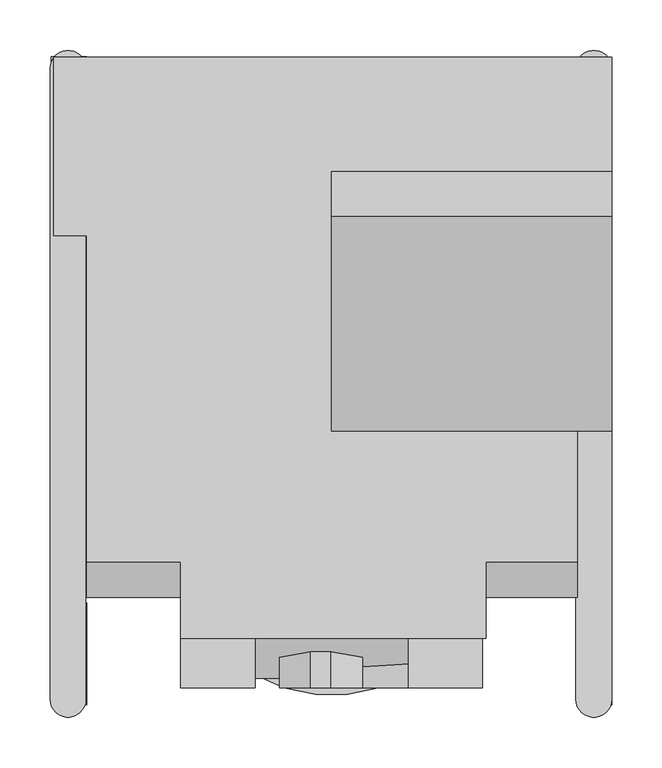
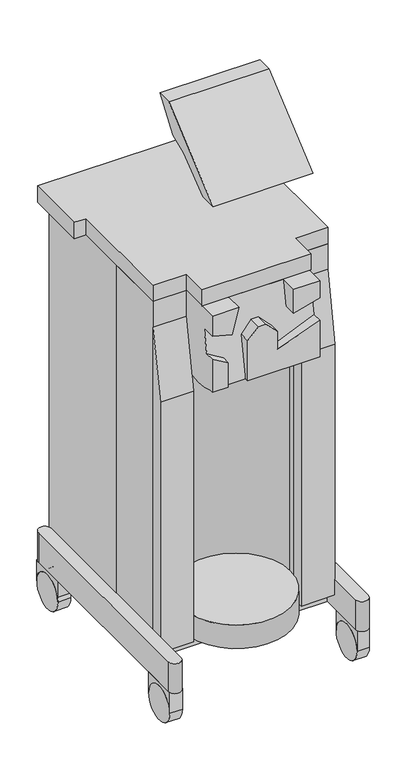
"""IFC4 building model written with IfcOpenShell, lengths in millimetres: proxy geometry, TB010 - CUSA : TB010 - CUSA."""

from ifc_helpers import new_model, si_unit, point, frame, frame_2d, origin, place, context, project, spatial, polyline, circle_curve, trimmed, segment, composite_curve, outline, extrude, faceted_brep, source, transform, mapped, element, save
from ifc_brep_helpers import plane_surface, cylinder_surface, revolved_surface, advanced_brep


def specialty_equipment_cd9e3837(model_context):
    return source(origin(), model_context, "Body", "SolidModel", [
        advanced_brep(
        [(31.190048, -304.8, 1006.9380598), (31.190048, -304.8, 1060.4753847), (-0.5345673, -304.8, 1092.2), (-21.0690363, -304.8, 1092.2), (-51.8302413, -304.8, 1061.4387949), (-51.8302413, -304.8, 943.2729477), (150.5310109, -304.8, 943.2729477), (150.5310109, -304.8, 1050.374618), (31.190048, -283.9074285, 1006.9380598), (31.190048, -274.4673537, 1060.4753847), (-0.5345673, -268.873448, 1092.2), (-21.0690363, -268.873448, 1092.2), (-51.8302413, -274.2974784, 1061.4387949), (-51.8302413, -295.1333055, 943.2729477), (150.5310109, -295.1333055, 943.2729477), (150.5310109, -179.2373321, 943.2729477), (150.5310109, -179.2373321, 1168.4), (150.5310109, -304.8, 1168.4), (150.5310109, -304.8, 1117.6), (150.5310109, -264.3947427, 1117.6), (150.5310109, -276.2483913, 1050.374618), (-150.5310109, -179.2373321, 1168.4), (-150.5310109, -179.2373321, 943.2729477), (-150.5310109, -295.1333055, 943.2729477), (-150.5310109, -304.8, 943.2729477), (-150.5310109, -304.8, 1041.4), (-150.5310109, -277.8308586, 1041.4), (-150.5310109, -265.83553, 1109.4288894), (-150.5310109, -304.8, 1109.4288894), (-150.5310109, -304.8, 1168.4), (76.9274629, -267.8722654, 1097.8779888), (76.9274629, -255.4373321, 1168.4), (-76.2, -255.4373321, 1168.4), (-95.9220112, -268.4156235, 1094.796452), (-106.5369204, -282.309564, 1016.0), (-106.5369204, -295.1333055, 943.2729477), (-76.2, -304.8, 1168.4), (76.9274629, -304.8, 1168.4), (76.9274629, -304.8, 1097.8779888), (-95.9220112, -304.8, 1094.796452), (-106.5369204, -304.8, 1016.0), (-106.5369204, -304.8, 943.2729477)],
        [
            (0, 1),
            (1, 2),
            (2, 3),
            (3, 4),
            (4, 5),
            (5, 6),
            (6, 7),
            (7, 0),
            (0, 8),
            (8, 9),
            (9, 1),
            (9, 10),
            (10, 2),
            (10, 11),
            (11, 3),
            (11, 12),
            (12, 4),
            (12, 13),
            (13, 5),
            (13, 14),
            (14, 6),
            (14, 15, circle_curve(frame((150.5310109, -237.1853188, 1091.5120177), z_axis=(1.0, 0.0, 0.0), x_axis=(0.0, 1.0, 0.0)), 159.1627816)),
            (15, 16),
            (16, 17),
            (17, 18),
            (18, 19),
            (19, 20),
            (20, 7),
            (20, 8),
            (21, 22),
            (22, 23, circle_curve(frame((-150.5310109, -237.1853188, 1091.5120177), z_axis=(-1.0, 0.0, 0.0), x_axis=(0.0, 1.0, 0.0)), 159.1627816)),
            (23, 24),
            (24, 25),
            (25, 26),
            (26, 27),
            (27, 28),
            (28, 29),
            (29, 21),
            (19, 30),
            (30, 31),
            (31, 32),
            (32, 33),
            (33, 27),
            (26, 34),
            (34, 35),
            (35, 13),
            (35, 23),
            (22, 15),
            (21, 16),
            (29, 36),
            (36, 32),
            (31, 37),
            (37, 17),
            (38, 18),
            (37, 38),
            (38, 30),
            (39, 36),
            (28, 39),
            (39, 33),
            (40, 25),
            (24, 41),
            (41, 40),
            (40, 34),
            (35, 41),
        ],
        [
            plane_surface(frame((31.190048, -304.8, 1006.9380598), z_axis=(0.0, -1.0, 0.0), x_axis=(0.0, 0.0, 1.0))),
            plane_surface(frame((31.190048, -304.8, 1006.9380598), z_axis=(1.0, 0.0, 0.0), x_axis=(0.0, 1.0, 0.0))),
            plane_surface(frame((31.190048, -304.8, 1060.4753847), z_axis=(0.7071067811865496, 0.0, 0.7071067811865456), x_axis=(0.0, 1.0, 0.0))),
            plane_surface(frame((-0.5345673, -304.8, 1092.2), z_axis=(0.0, 0.0, 1.0), x_axis=(0.0, 1.0, 0.0))),
            plane_surface(frame((-21.0690363, -304.8, 1092.2), z_axis=(-0.707106781186545, 0.0, 0.7071067811865501), x_axis=(0.0, 1.0, 0.0))),
            plane_surface(frame((-51.8302413, -304.8, 1061.4387949), z_axis=(-1.0, 0.0, 0.0), x_axis=(0.0, 1.0, 0.0))),
            plane_surface(frame((-51.8302413, -304.8, 943.2729477), z_axis=(0.0, 0.0, -1.0), x_axis=(0.0, 1.0, 0.0))),
            plane_surface(frame((150.5310109, -304.8, 943.2729477), z_axis=(1.0, 0.0, 0.0), x_axis=(0.0, 1.0, 0.0))),
            plane_surface(frame((150.5310109, -304.8, 1050.374618), z_axis=(-0.3420201433256685, 0.0, 0.9396926207859085), x_axis=(0.0, 1.0, 0.0))),
            plane_surface(frame((-150.5310109, -255.4373321, 1168.4), z_axis=(-1.0, 0.0, 0.0), x_axis=(0.0, 0.17364817766693152, 0.9848077530122079))),
            plane_surface(frame((150.5310109, -255.4373321, 1168.4), z_axis=(0.0, -0.9848077530122079, 0.17364817766693152), x_axis=(-1.0, 0.0, 0.0))),
            cylinder_surface(frame((-150.5310109, -237.1853188, 1091.5120177), z_axis=(1.0, 0.0, 0.0), x_axis=(0.0, 1.0, 0.0)), 159.1627816),
            plane_surface(frame((150.5310109, -179.2373321, 943.2729477), z_axis=(0.0, 1.0, 0.0), x_axis=(-1.0, 0.0, 0.0))),
            plane_surface(frame((150.5310109, -179.2373321, 1168.4), z_axis=(0.0, 0.0, 1.0), x_axis=(-1.0, 0.0, 0.0))),
            plane_surface(frame((150.5310109, -304.8, 1117.6), z_axis=(0.0, -1.0000000000000002, 0.0), x_axis=(0.9659258262890681, 0.0, 0.2588190451025219))),
            plane_surface(frame((76.9274629, -304.8, 1097.8779888), z_axis=(0.2588190451025219, 0.0, -0.9659258262890681), x_axis=(0.0, 1.0, 0.0))),
            plane_surface(frame((76.9274629, -304.8, 1168.4), z_axis=(-1.0, 0.0, 0.0), x_axis=(0.0, 1.0, 0.0))),
            plane_surface(frame((-76.2, -304.8, 1168.4), z_axis=(0.0, -1.0000000000000002, 0.0), x_axis=(0.2588190451025218, 0.0, 0.9659258262890681))),
            plane_surface(frame((-95.9220112, -304.8, 1094.796452), z_axis=(0.9659258262890681, 0.0, -0.2588190451025218), x_axis=(0.0, 1.0, 0.0))),
            plane_surface(frame((-150.5310109, -304.8, 1109.4288894), z_axis=(-0.25881904510252624, 0.0, -0.9659258262890669), x_axis=(0.0, 1.0, 0.0))),
            plane_surface(frame((-150.5310109, -304.8, 1041.4), z_axis=(0.0, -1.0, 0.0), x_axis=(-0.8660254037844382, 0.0, 0.5000000000000009))),
            plane_surface(frame((-106.5369204, -304.8, 1016.0), z_axis=(0.5000000000000009, 0.0, 0.8660254037844382), x_axis=(0.0, 1.0, 0.0))),
            plane_surface(frame((-150.5310109, -304.8, 943.2729477), z_axis=(0.0, 0.0, -1.0), x_axis=(0.0, 1.0, 0.0))),
            plane_surface(frame((-106.5369204, -304.8, 943.2729477), z_axis=(1.0, 0.0, 0.0), x_axis=(0.0, 1.0, 0.0))),
        ],
        [
            (0, [[1, 2, 3, 4, 5, 6, 7, 8]]),
            (1, [[-1, 9, 10, 11]]),
            (2, [[-2, -11, 12, 13]]),
            (3, [[-3, -13, 14, 15]]),
            (4, [[-4, -15, 16, 17]]),
            (5, [[-5, -17, 18, 19]]),
            (6, [[-6, -19, 20, 21]]),
            (7, [[-7, -21, 22, 23, 24, 25, 26, 27, 28]]),
            (8, [[-8, -28, 29, -9]]),
            (9, [[30, 31, 32, 33, 34, 35, 36, 37, 38]]),
            (10, [[-10, -29, -27, 39, 40, 41, 42, 43, -35, 44, 45, 46, -18, -16, -14, -12]]),
            (11, [[-22, -20, -46, 47, -31, 48]]),
            (12, [[-23, -48, -30, 49]]),
            (13, [[-49, -38, 50, 51, -41, 52, 53, -24]]),
            (14, [[54, -25, -53, 55]]),
            (15, [[-54, 56, -39, -26]]),
            (16, [[-55, -52, -40, -56]]),
            (17, [[57, -50, -37, 58]]),
            (18, [[-57, 59, -42, -51]]),
            (19, [[-58, -36, -43, -59]]),
            (20, [[60, -33, 61, 62]]),
            (21, [[-60, 63, -44, -34]]),
            (22, [[-61, -32, -47, 64]]),
            (23, [[-62, -64, -45, -63]]),
        ],
    ),
        faceted_brep([(279.4, 146.05, 1377.95), (279.4, 209.9575289, 1464.1268053), (279.4, 165.5075289, 1464.1268053), (279.4, -48.5252886, 1284.5319471), (279.4, 0.0, 1284.5319471), (279.4, 95.25, 1356.3079704), (279.4, 95.25, 1270.0), (279.4, 146.05, 1270.0), (0.0, 95.25, 1356.3079704), (0.0, 0.0, 1284.5319471), (0.0, -48.5252886, 1284.5319471), (0.0, 165.5075289, 1464.1268053), (0.0, 209.9575289, 1464.1268053), (0.0, 146.05, 1377.95), (245.3601172, 146.05, 1377.95), (245.3601172, 95.25, 1356.3079704), (245.3601172, 95.25, 1270.0), (245.3601172, 146.05, 1270.0)], [[[0, 1, 2, 3, 4, 5, 6, 7]], [[8, 9, 10, 11, 12, 13]], [[1, 0, 14, 13, 12]], [[2, 1, 12, 11]], [[3, 2, 11, 10]], [[4, 3, 10, 9]], [[5, 4, 9, 8, 15]], [[6, 5, 15, 16]], [[7, 6, 16, 17]], [[0, 7, 17, 14]], [[15, 14, 17, 16]], [[14, 15, 8, 13]]]),
        extrude(outline(polyline([(279.4, 146.05), (279.4, 95.25), (245.3601172, 95.25), (245.3601172, 146.05), (279.4, 146.05)])), frame((0.0, 0.0, 1168.4), z_axis=(0.0, 0.0, 1.0), x_axis=(1.0, 0.0, 0.0)), (0.0, 0.0, 1.0), 101.6),
        extrude(outline(polyline([(-150.5310109, -179.2373321), (-243.8144634, -179.2373321), (-243.8144634, 146.05), (-276.7922586, 146.05), (-276.7922586, 323.85), (279.4, 323.85), (279.4, 150.9626679), (245.3601172, 150.9626679), (245.3601172, -179.2373321), (154.2689891, -179.2373321), (154.2689891, -255.4373321), (-150.5310109, -255.4373321), (-150.5310109, -179.2373321)])), frame((0.0, 0.0, 1168.4), z_axis=(0.0, 0.0, 1.0), x_axis=(1.0, 0.0, 0.0)), (0.0, 0.0, 1.0), 47.9518791),
        extrude(outline(polyline([(-214.5226418, 892.0870646), (-179.2373321, 1092.2), (-179.2373321, 151.1568458), (-214.5226418, 151.1568458), (-214.5226418, 892.0870646)])), frame((-243.8144634, 0.0, 0.0), z_axis=(1.0, 0.0, 0.0), x_axis=(0.0, 1.0, 0.0)), (0.0, 0.0, 1.0), 93.2834525),
        extrude(outline(polyline([(-214.5226418, 892.0870646), (-179.2373321, 1092.2), (-179.2373321, 151.1568458), (-214.5226418, 151.1568458), (-214.5226418, 892.0870646)])), frame((150.5310109, 0.0, 0.0), z_axis=(1.0, 0.0, 0.0), x_axis=(0.0, 1.0, 0.0)), (0.0, 0.0, 1.0), 94.8291063),
        extrude(outline(composite_curve([segment(trimmed(circle_curve(frame_2d((0.0, -159.5597323)), 152.4), [point((-152.4, -159.5597323))], [point((152.4, -159.5597323))], False, "CARTESIAN"), True, "CONTINUOUS"), segment(trimmed(circle_curve(frame_2d((0.0, -159.5597323)), 152.4), [point((152.4, -159.5597323))], [point((-152.4, -159.5597323))], False, "CARTESIAN"), True, "CONTINUOUS")], self_intersect=False)), frame((0.0, 0.0, 151.1568458), z_axis=(0.0, 0.0, 1.0), x_axis=(1.0, 0.0, 0.0)), (0.0, 0.0, 1.0), 69.4082655),
        advanced_brep(
        [(-243.8144634, 323.85, 1168.4), (-243.8144634, 0.0, 1168.4), (-243.8144634, -179.2373321, 1168.4), (245.3601172, -179.2373321, 1168.4), (245.3601172, 323.85, 1168.4), (-243.8144634, 323.85, 111.211617), (245.3601172, 323.85, 111.211617), (245.3601172, -179.2373321, 111.211617), (-243.8144634, -179.2373321, 111.211617), (-243.8144634, 0.0, 111.211617), (-150.5310109, -179.2373321, 938.5718948), (150.5310109, -179.2373321, 938.5718948), (150.5310109, -179.2373321, 199.0338376), (-150.5310109, -179.2373321, 199.0338376), (-152.4, -155.442905, 938.5718948), (152.4, -155.442905, 938.5718948), (152.4, -155.442905, 199.0338376), (-152.4, -155.442905, 199.0338376)],
        [
            (0, 1),
            (1, 2),
            (2, 3),
            (3, 4),
            (4, 0),
            (5, 6),
            (6, 7),
            (7, 8),
            (8, 9),
            (9, 5),
            (0, 5),
            (9, 1),
            (8, 2),
            (7, 3),
            (10, 11),
            (11, 12),
            (12, 13),
            (13, 10),
            (6, 4),
            (14, 15, circle_curve(frame((0.0, -155.442905, 938.5718948), z_axis=(0.0, 0.0, -1.0), x_axis=(1.0, 0.0, 0.0)), 152.4)),
            (15, 11, circle_curve(frame((0.0, -155.442905, 938.5718948), z_axis=(0.0, 0.0, -1.0), x_axis=(1.0, 0.0, 0.0)), 152.4)),
            (10, 14, circle_curve(frame((0.0, -155.442905, 938.5718948), z_axis=(0.0, 0.0, -1.0), x_axis=(1.0, 0.0, 0.0)), 152.4)),
            (16, 17, circle_curve(frame((0.0, -155.442905, 199.0338376), z_axis=(0.0, 0.0, 1.0), x_axis=(1.0, 0.0, 0.0)), 152.4)),
            (17, 13, circle_curve(frame((0.0, -155.442905, 199.0338376), z_axis=(0.0, 0.0, 1.0), x_axis=(1.0, 0.0, 0.0)), 152.4)),
            (12, 16, circle_curve(frame((0.0, -155.442905, 199.0338376), z_axis=(0.0, 0.0, 1.0), x_axis=(1.0, 0.0, 0.0)), 152.4)),
            (15, 16),
            (17, 14),
        ],
        [
            plane_surface(frame((-243.8144634, 0.0, 1168.4), z_axis=(0.0, 0.0, 1.0), x_axis=(0.0, -1.0, 0.0))),
            plane_surface(frame((-243.8144634, 0.0, 111.211617), z_axis=(0.0, 0.0, -1.0), x_axis=(0.0, 1.0, 0.0))),
            plane_surface(frame((-243.8144634, 323.85, 1168.4), z_axis=(-1.0, 0.0, 0.0), x_axis=(0.0, 0.0, -1.0))),
            plane_surface(frame((-243.8144634, 0.0, 1168.4), z_axis=(-1.0, 0.0, 0.0), x_axis=(0.0, 0.0, -1.0))),
            plane_surface(frame((-243.8144634, -179.2373321, 1168.4), z_axis=(0.0, -1.0, 0.0), x_axis=(0.0, 0.0, -1.0))),
            plane_surface(frame((245.3601172, -179.2373321, 1168.4), z_axis=(1.0, 0.0, 0.0), x_axis=(0.0, 0.0, -1.0))),
            plane_surface(frame((245.3601172, 323.85, 1168.4), z_axis=(0.0, 1.0, 0.0), x_axis=(0.0, 0.0, -1.0))),
            plane_surface(frame((152.4, -155.442905, 938.5718948), z_axis=(0.0, 0.0, -1.0), x_axis=(0.0, 1.0, 0.0))),
            plane_surface(frame((152.4, -155.442905, 199.0338376), z_axis=(0.0, 0.0, 1.0), x_axis=(0.0, -1.0, 0.0))),
            revolved_surface(polyline([(152.4, -155.442905, 938.5718948), (152.4, -155.442905, 199.0338376)]), (0.0, -155.442905, 199.0338376), (0.0, 0.0, 1.0)),
        ],
        [
            (0, [[1, 2, 3, 4, 5]]),
            (1, [[6, 7, 8, 9, 10]]),
            (2, [[-1, 11, -10, 12]]),
            (3, [[-2, -12, -9, 13]]),
            (4, [[-3, -13, -8, 14], [15, 16, 17, 18]]),
            (5, [[-4, -14, -7, 19]]),
            (6, [[-5, -19, -6, -11]]),
            (7, [[20, 21, -15, 22]]),
            (8, [[23, 24, -17, 25]]),
            (9, [[26, -25, -16, -21]]),
            (9, [[27, -22, -18, -24]]),
            (9, [[-20, -27, -23, -26]]),
        ],
    ),
        extrude(outline(composite_curve([segment(trimmed(circle_curve(frame_2d((273.6915531, 49.551594)), 50.8), [point((324.4915531, 49.551594))], [point((222.8915531, 49.551594))], True, "CARTESIAN"), True, "CONTINUOUS"), segment(polyline([(222.8915531, 49.551594), (222.8915531, 111.211617), (324.4915531, 111.211617), (324.4915531, 49.551594)]), True, "CONTINUOUS")], self_intersect=False)), frame((-279.4, 0.0, 0.0), z_axis=(1.0, 0.0, 0.0), x_axis=(0.0, 1.0, 0.0)), (0.0, 0.0, 1.0), 35.5855366),
        advanced_brep(
        [(-243.8144634, -219.9479579, 49.551594), (-243.8144634, -219.9479579, 111.211617), (-243.8144634, -321.5479579, 111.211617), (-243.8144634, -321.5479579, 49.551594), (-279.4, -219.9479579, 49.551594), (-279.4, -321.5479579, 49.551594), (-279.4, -321.5479579, 111.211617), (-279.4, -219.9479579, 111.211617)],
        [
            (0, 1),
            (1, 2),
            (2, 3),
            (3, 0, circle_curve(frame((-243.8144634, -270.7479579, 49.551594), z_axis=(-1.0, 0.0, 0.0), x_axis=(0.0, 1.0, 0.0)), 50.8)),
            (4, 5, circle_curve(frame((-279.4, -270.7479579, 49.551594), z_axis=(1.0, 0.0, 0.0), x_axis=(0.0, 1.0, 0.0)), 50.8)),
            (5, 6),
            (6, 7),
            (7, 4),
            (0, 4),
            (7, 1),
            (6, 2),
            (5, 3),
        ],
        [
            plane_surface(frame((-243.8144634, -219.9479579, 49.551594), z_axis=(1.0, 0.0, 0.0), x_axis=(0.0, 0.0, 1.0))),
            plane_surface(frame((-279.4, -219.9479579, 49.551594), z_axis=(-1.0, 0.0, 0.0), x_axis=(0.0, 0.0, -1.0))),
            plane_surface(frame((-243.8144634, -219.9479579, 49.551594), z_axis=(0.0, 1.0, 0.0), x_axis=(-1.0, 0.0, 0.0))),
            plane_surface(frame((-243.8144634, -219.9479579, 111.211617), z_axis=(0.0, 0.0, 1.0), x_axis=(-1.0, 0.0, 0.0))),
            plane_surface(frame((-243.8144634, -321.5479579, 111.211617), z_axis=(0.0, -1.0, 0.0), x_axis=(-1.0, 0.0, 0.0))),
            revolved_surface(polyline([(-279.4, -219.9479579, 49.551594), (-243.8144634, -219.9479579, 49.551594)]), (-279.4, -270.7479579, 49.551594), (-1.0, 0.0, 0.0)),
        ],
        [
            (0, [[1, 2, 3, 4]]),
            (1, [[5, 6, 7, 8]]),
            (2, [[-1, 9, -8, 10]]),
            (3, [[-2, -10, -7, 11]]),
            (4, [[-3, -11, -6, 12]]),
            (5, [[-4, -12, -5, -9]]),
        ],
    ),
        advanced_brep(
        [(279.4, -219.9479579, 49.551594), (279.4, -219.9479579, 111.211617), (279.4, 222.25, 111.211617), (279.4, 222.25, 49.551594), (279.4, 323.85, 49.551594), (279.4, 323.85, 111.211617), (279.4, 313.0782408, 111.211617), (279.4, 313.0782408, 199.0338376), (279.4, -316.2669769, 199.0338376), (279.4, -316.2669769, 111.211617), (279.4, -321.5479579, 111.211617), (279.4, -321.5479579, 49.551594), (245.3601172, -219.9479579, 49.551594), (245.3601172, -321.5479579, 49.551594), (245.3601172, -321.5479579, 111.211617), (245.3601172, -219.9479579, 111.211617), (278.5982247, -321.5479579, 111.211617), (243.8144634, 313.0782408, 199.0338376), (243.8144634, -316.2669769, 199.0338376), (243.8144634, -316.2669769, 111.211617), (243.8144634, 313.0782408, 111.211617), (245.3601172, 320.331783, 111.211617), (245.3601172, 222.25, 111.211617), (247.4456001, 323.85, 111.211617), (275.7688632, 323.85, 111.211617), (245.3601172, 323.85, 49.551594), (245.3601172, 222.25, 49.551594), (245.3601172, 323.85, 111.211617)],
        [
            (0, 1),
            (1, 2),
            (2, 3),
            (3, 4, circle_curve(frame((279.4, 273.05, 49.551594), z_axis=(-1.0, 0.0, 0.0), x_axis=(0.0, 1.0, 0.0)), 50.8)),
            (4, 5),
            (5, 6),
            (6, 7),
            (7, 8),
            (8, 9),
            (9, 10),
            (10, 11),
            (11, 0, circle_curve(frame((279.4, -270.7479579, 49.551594), z_axis=(-1.0, 0.0, 0.0), x_axis=(0.0, 1.0, 0.0)), 50.8)),
            (12, 13, circle_curve(frame((245.3601172, -270.7479579, 49.551594), z_axis=(1.0, 0.0, 0.0), x_axis=(0.0, 1.0, 0.0)), 50.8)),
            (13, 14),
            (14, 15),
            (15, 12),
            (0, 12),
            (15, 1),
            (9, 16, circle_curve(frame((261.6072317, -316.2669769, 111.211617), z_axis=(0.0, 0.0, -1.0), x_axis=(1.0, 0.0, 0.0)), 17.7927683)),
            (16, 10),
            (16, 14),
            (13, 11),
            (7, 17, circle_curve(frame((261.6072317, 313.0782408, 199.0338376), z_axis=(0.0, 0.0, 1.0), x_axis=(1.0, 0.0, 0.0)), 17.7927683)),
            (17, 18),
            (18, 8, circle_curve(frame((261.6072317, -316.2669769, 199.0338376), z_axis=(0.0, 0.0, 1.0), x_axis=(1.0, 0.0, 0.0)), 17.7927683)),
            (19, 20),
            (20, 21, circle_curve(frame((261.6072317, 313.0782408, 111.211617), z_axis=(0.0, 0.0, -1.0), x_axis=(1.0, 0.0, 0.0)), 17.7927683)),
            (21, 22),
            (22, 2),
            (16, 19, circle_curve(frame((261.6072317, -316.2669769, 111.211617), z_axis=(0.0, 0.0, -1.0), x_axis=(1.0, 0.0, 0.0)), 17.7927683)),
            (23, 24, circle_curve(frame((261.6072317, 313.0782408, 111.211617), z_axis=(0.0, 0.0, -1.0), x_axis=(1.0, 0.0, 0.0)), 17.7927683)),
            (24, 23),
            (6, 24, circle_curve(frame((261.6072317, 313.0782408, 111.211617), z_axis=(0.0, 0.0, 1.0), x_axis=(1.0, 0.0, 0.0)), 17.7927683)),
            (23, 21, circle_curve(frame((261.6072317, 313.0782408, 111.211617), z_axis=(0.0, 0.0, 1.0), x_axis=(1.0, 0.0, 0.0)), 17.7927683)),
            (20, 17),
            (19, 18),
            (25, 26, circle_curve(frame((245.3601172, 273.05, 49.551594), z_axis=(1.0, 0.0, 0.0), x_axis=(0.0, 1.0, 0.0)), 50.8)),
            (26, 22),
            (21, 27),
            (27, 25),
            (4, 25),
            (27, 23),
            (24, 5),
            (26, 3),
        ],
        [
            plane_surface(frame((279.4, -219.9479579, 49.551594), z_axis=(1.0, 0.0, 0.0), x_axis=(0.0, 0.0, 1.0))),
            plane_surface(frame((245.3601172, -219.9479579, 49.551594), z_axis=(-1.0, 0.0, 0.0), x_axis=(0.0, 0.0, -1.0))),
            plane_surface(frame((279.4, -219.9479579, 49.551594), z_axis=(0.0, 1.0, 0.0), x_axis=(-1.0, 0.0, 0.0))),
            plane_surface(frame((279.4, -219.9479579, 111.211617), z_axis=(0.0, 0.0, 1.0), x_axis=(-1.0, 0.0, 0.0))),
            plane_surface(frame((279.4, -321.5479579, 111.211617), z_axis=(0.0, -1.0, 0.0), x_axis=(-1.0, 0.0, 0.0))),
            revolved_surface(polyline([(245.3601172, -219.9479579, 49.551594), (279.4, -219.9479579, 49.551594)]), (245.3601172, -270.7479579, 49.551594), (-1.0, 0.0, 0.0)),
            plane_surface(frame((279.4, 298.45, 199.0338376), z_axis=(0.0, 0.0, 1.0), x_axis=(0.0, 1.0, 0.0))),
            plane_surface(frame((279.4, 298.45, 111.211617), z_axis=(0.0, 0.0, -1.0), x_axis=(0.0, -1.0, 0.0))),
            cylinder_surface(frame((261.6072317, 313.0782408, 111.211617), z_axis=(0.0, 0.0, 1.0), x_axis=(1.0, 0.0, 0.0)), 17.7927683),
            plane_surface(frame((243.8144634, 313.0782408, 199.0338376), z_axis=(-1.0, 0.0, 0.0), x_axis=(0.0, 0.0, -1.0))),
            cylinder_surface(frame((261.6072317, -316.2669769, 111.211617), z_axis=(0.0, 0.0, 1.0), x_axis=(1.0, 0.0, 0.0)), 17.7927683),
            plane_surface(frame((245.3601172, 323.85, 49.551594), z_axis=(-1.0, 0.0, 0.0), x_axis=(0.0, 0.0, -1.0))),
            plane_surface(frame((279.4, 323.85, 49.551594), z_axis=(0.0, 1.0, 0.0), x_axis=(-1.0, 0.0, 0.0))),
            plane_surface(frame((279.4, 323.85, 111.211617), z_axis=(0.0, 0.0, 1.0), x_axis=(-1.0, 0.0, 0.0))),
            plane_surface(frame((279.4, 222.25, 111.211617), z_axis=(0.0, -1.0, 0.0), x_axis=(-1.0, 0.0, 0.0))),
            revolved_surface(polyline([(245.3601172, 323.85, 49.551594), (279.4, 323.85, 49.551594)]), (245.3601172, 273.05, 49.551594), (-1.0, 0.0, 0.0)),
        ],
        [
            (0, [[1, 2, 3, 4, 5, 6, 7, 8, 9, 10, 11, 12]]),
            (1, [[13, 14, 15, 16]]),
            (2, [[-1, 17, -16, 18]]),
            (3, [[-10, 19, 20]]),
            (4, [[-11, -20, 21, -14, 22]]),
            (5, [[-12, -22, -13, -17]]),
            (6, [[-8, 23, 24, 25]]),
            (7, [[26, 27, 28, 29, -2, -18, -15, -21, 30]]),
            (7, [[31, 32]]),
            (8, [[-23, -7, 33, -31, 34, -27, 35]]),
            (9, [[-24, -35, -26, 36]]),
            (10, [[-25, -36, -30, -19, -9]]),
            (11, [[37, 38, -28, 39, 40]]),
            (12, [[-5, 41, -40, 42, -32, 43]]),
            (13, [[-6, -43, -33]]),
            (13, [[-39, -34, -42]]),
            (14, [[-3, -29, -38, 44]]),
            (15, [[-4, -44, -37, -41]]),
        ],
    ),
        extrude(outline(composite_curve([segment(trimmed(circle_curve(frame_2d((-262.6306271, -316.2669769)), 17.7927683), [point((-244.8378587, -316.2669769))], [point((-280.4233954, -316.2669769))], False, "CARTESIAN"), True, "CONTINUOUS"), segment(polyline([(-280.4233954, -316.2669769), (-280.4233954, 313.0782408)]), True, "CONTINUOUS"), segment(trimmed(circle_curve(frame_2d((-262.6306271, 313.0782408)), 17.7927683), [point((-280.4233954, 313.0782408))], [point((-244.8378587, 313.0782408))], False, "CARTESIAN"), True, "CONTINUOUS"), segment(polyline([(-244.8378587, 313.0782408), (-244.8378587, -316.2669769)]), True, "CONTINUOUS")], self_intersect=False)), frame((0.0, 0.0, 111.211617), z_axis=(0.0, 0.0, 1.0), x_axis=(1.0, 0.0, 0.0)), (0.0, 0.0, 1.0), 87.8222206),
        extrude(outline(composite_curve([segment(trimmed(circle_curve(frame_2d((-270.7479579, 49.551594)), 50.8), [point((-321.5479579, 49.551594))], [point((-219.9479579, 49.551594))], False, "CARTESIAN"), True, "CONTINUOUS"), segment(trimmed(circle_curve(frame_2d((-270.7479579, 49.551594)), 50.8), [point((-219.9479579, 49.551594))], [point((-321.5479579, 49.551594))], False, "CARTESIAN"), True, "CONTINUOUS")], self_intersect=False)), frame((-279.4, 0.0, 0.0), z_axis=(1.0, 0.0, 0.0), x_axis=(0.0, 1.0, 0.0)), (0.0, 0.0, 1.0), 35.5855366),
        extrude(outline(composite_curve([segment(trimmed(circle_curve(frame_2d((271.5158223, 49.551594)), 50.8), [point((220.7158223, 49.551594))], [point((322.3158223, 49.551594))], False, "CARTESIAN"), True, "CONTINUOUS"), segment(trimmed(circle_curve(frame_2d((271.5158223, 49.551594)), 50.8), [point((322.3158223, 49.551594))], [point((220.7158223, 49.551594))], False, "CARTESIAN"), True, "CONTINUOUS")], self_intersect=False)), frame((-279.4, 0.0, 0.0), z_axis=(1.0, 0.0, 0.0), x_axis=(0.0, 1.0, 0.0)), (0.0, 0.0, 1.0), 35.5855366),
        extrude(outline(composite_curve([segment(trimmed(circle_curve(frame_2d((-270.7479579, 49.551594)), 50.8), [point((-321.5479579, 49.551594))], [point((-219.9479579, 49.551594))], False, "CARTESIAN"), True, "CONTINUOUS"), segment(trimmed(circle_curve(frame_2d((-270.7479579, 49.551594)), 50.8), [point((-219.9479579, 49.551594))], [point((-321.5479579, 49.551594))], False, "CARTESIAN"), True, "CONTINUOUS")], self_intersect=False)), frame((245.3601172, 0.0, 0.0), z_axis=(1.0, 0.0, 0.0), x_axis=(0.0, 1.0, 0.0)), (0.0, 0.0, 1.0), 34.0398828),
        extrude(outline(composite_curve([segment(trimmed(circle_curve(frame_2d((271.5158223, 49.551594)), 50.8), [point((220.7158223, 49.551594))], [point((322.3158223, 49.551594))], False, "CARTESIAN"), True, "CONTINUOUS"), segment(trimmed(circle_curve(frame_2d((271.5158223, 49.551594)), 50.8), [point((322.3158223, 49.551594))], [point((220.7158223, 49.551594))], False, "CARTESIAN"), True, "CONTINUOUS")], self_intersect=False)), frame((245.3601172, 0.0, 0.0), z_axis=(1.0, 0.0, 0.0), x_axis=(0.0, 1.0, 0.0)), (0.0, 0.0, 1.0), 34.0398828),
    ])


if __name__ == "__main__":
    model = new_model("IFC4")
    model_context = context("Model", 3, world=origin())
    ifc_project = project(units=[si_unit("LENGTHUNIT", "METRE", prefix="MILLI")], contexts=[model_context])
    site = spatial("IfcSite", under=ifc_project)
    building = spatial("IfcBuilding", under=site)
    placement = place(None, origin())
    specialty_equipment_shape = specialty_equipment_cd9e3837(model_context)
    element("IfcBuildingElementProxy", 1, Name="TB010 - CUSA : TB010 - CUSA", ObjectType="TB010 - CUSA : TB010 - CUSA", at=placement, inside=building, context=model_context, shape_type="MappedRepresentation", body=[
        mapped(specialty_equipment_shape, transform((0.0, 0.0, 0.0), x_axis=(1.0, 0.0, 0.0), y_axis=(0.0, 1.0, 0.0), z_axis=(0.0, 0.0, 1.0))),
    ])
    save(model, "model.ifc")

# Revit data of these elements
# Type "TB010 - CUSA : TB010 - CUSA"
#   Watts2 = "0"
#   Watts1 = "0"
#   Unit_Issue = "EA"
#   UTIL_6_Misc = "-"
#   UTIL_5_NonMedGas = "-"
#   UTIL_4_MiscGas = "-"
#   UTIL_3_MedGas = "-"
#   UTIL_2_Elec = "-"
#   UTIL_1_WaterDrain = "-"
#   Nomenclature = "CUSA"
#   NSN = ""
#   Location [instance default] = ""
#   JSN = "TB010"
#   Fund_Source_VA = "-"
#   Fund_Source_Navy = "-"
#   Fund_Source_Army = "-"
#   Fund_Source_AF = "-"
#   ELEC_Volts2 = "0"
#   ELEC_Volts1 = "0"
#   ELEC_Phase2 = "0"
#   ELEC_Phase1 = "0"
#   ELEC_HertzSwitch = "0"
#   ELEC_HertzDependent = "0"
#   ELEC_Hertz = "0"
#   ELEC_Amps2 = "0"
#   ELEC_Amps1 = "0"
#   DetailDescription = ""
#   CAT_VA = "C"
#   CAT_Navy = "C"
#   CAT_IHS = "-"
#   CAT_Army = "C"
#   CAT_AF = "C"
#   BTUperhour = "0"
#   Weight_IP = 0
#   DIM_Width_IP = 1' - 10"
#   DIM_Height_IP = 3' - 10"
#   DIM_Depth_IP = 2' - 1 1/2"
# Element 1 (IfcBuildingElementProxy, "TB010 - CUSA : TB010 - CUSA")
#   Materials on its faces: "Default"
# Materials
#   "Default": class "Miscellaneous", colour RGB 127 127 127, transparency 0
